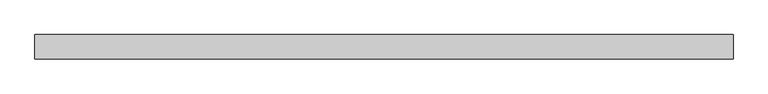
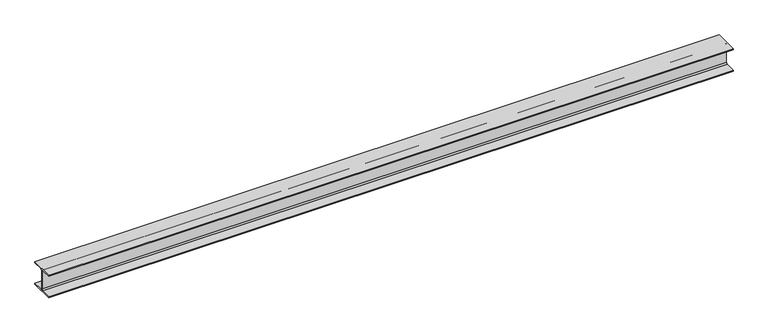
"""IFC4 building model written with IfcOpenShell, lengths in millimetres: beam geometry, 0912_Steel Framing_H-KSD3502 : H_SB_ASB_H-300x300x10x15."""

from ifc_helpers import new_model, si_unit, point, frame, frame_2d, origin, place, context, project, spatial, polyline, circle_curve, trimmed, segment, composite_curve, outline, extrude, source, transform, mapped, element, save


def beam_92893fa5(model_context):
    return source(origin(), model_context, "Body", "SweptSolid", [
        extrude(outline(composite_curve([segment(polyline([(150.0, -135.0), (150.0, -150.0), (-150.0, -150.0), (-150.0, -135.0), (-23.0, -135.0)]), True, "CONTINUOUS"), segment(trimmed(circle_curve(frame_2d((-23.0, -117.0)), 18.0), [point((-23.0, -135.0))], [point((-5.0, -117.0))], True, "CARTESIAN"), True, "CONTINUOUS"), segment(polyline([(-5.0, -117.0), (-5.0, 117.0)]), True, "CONTINUOUS"), segment(trimmed(circle_curve(frame_2d((-23.0, 117.0)), 18.0), [point((-5.0, 117.0))], [point((-23.0, 135.0))], True, "CARTESIAN"), True, "CONTINUOUS"), segment(polyline([(-23.0, 135.0), (-150.0, 135.0), (-150.0, 150.0), (150.0, 150.0), (150.0, 135.0), (23.0, 135.0)]), True, "CONTINUOUS"), segment(trimmed(circle_curve(frame_2d((23.0, 117.0)), 18.0), [point((23.0, 135.0))], [point((5.0, 117.0))], True, "CARTESIAN"), True, "CONTINUOUS"), segment(polyline([(5.0, 117.0), (5.0, -117.0)]), True, "CONTINUOUS"), segment(trimmed(circle_curve(frame_2d((23.0, -117.0)), 18.0), [point((5.0, -117.0))], [point((23.0, -135.0))], True, "CARTESIAN"), True, "CONTINUOUS"), segment(polyline([(23.0, -135.0), (150.0, -135.0)]), True, "CONTINUOUS")], self_intersect=False)), frame((-4331.4958952, 0.0, 0.0), z_axis=(1.0, 0.0, 0.0), x_axis=(0.0, 1.0, 0.0)), (0.0, 0.0, 1.0), 8594.5528849),
    ])


if __name__ == "__main__":
    model = new_model("IFC4")
    model_context = context("Model", 3, world=origin())
    ifc_project = project(units=[si_unit("LENGTHUNIT", "METRE", prefix="MILLI")], contexts=[model_context])
    site = spatial("IfcSite", under=ifc_project)
    building = spatial("IfcBuilding", under=site)
    placement = place(None, origin())
    beam_shape = beam_92893fa5(model_context)
    element("IfcBeam", 1, ObjectType="0912_Steel Framing_H-KSD3502 : H_SB_ASB_H-300x300x10x15", at=placement, inside=building, context=model_context, shape_type="MappedRepresentation", body=[
        mapped(beam_shape, transform((0.0, 0.0, 0.0), x_axis=(1.0, 0.0, 0.0), y_axis=(0.0, 1.0, 0.0), z_axis=(0.0, 0.0, 1.0))),
    ])
    save(model, "model.ifc")

# Revit data of these elements
# Type "0912_Steel Framing_H-KSD3502 : H_SB_ASB_H-300x300x10x15"
#   H_WM Code_1 = "S01AA001-00001 | Main Steel Structure Fabrication Work | Shelter/Building | Heavy Steel - Standard (Weight≥90KG/M) | Material: (   )"
#   H_WM Code_2 = "S03AA027-00001 | Main Steel Structure Erection Work | Shelter/Building | Heavy Steel (Weight≥90KG/M) | Material: (   )"
#   H_WM Code_3 = "S01AA010-00001 | Main Steel Structure Fabrication Work | Shelter/Building | Steel Painting/Coating | for Non-Fireproofed Steel Surface, Surface Preparation, Primer, Second & Final Coat | Material: (   )"
#   H_Q'ty Cal Type Tag = "SB-Q2"
#   Width = 30.0 cm
#   Web Thickness = 1.0 cm
#   Web Fillet = 1.8 cm
#   Warping Constant = 1370000.0 cm⁶
#   W = 0
#   Torsional Moment of Inertia = 77.00 cm⁴
#   Section Area = 119.8 cm²
#   Plastic Modulus weak axis = 684.0 cm³
#   Plastic Modulus strong axis = 1500.0 cm³
#   Perimeter = 1.75 m²/m
#   Nominal Weight = 94.00 kgf/m
#   Moment of Inertia weak axis = 6750.00 cm⁴
#   Moment of Inertia strong axis = 20400.00 cm⁴
#   Height = 30.0 cm
#   Flange Thickness = 1.5 cm
#   Elastic Modulus weak axis = 450.0 cm³
#   Elastic Modulus strong axis = 1360.0 cm³
#   Centroid Vertical = 15.0 cm
#   Centroid Horizontal = 15.0 cm
#   Ix = 204000000
#   Length [instance default] = 1.5240 m
#   Zx = 1500000
#   b = 0.3000 m
#   h = 0.3000 m
#   r = 0.0180 m
#   s = 0.0100 m
#   t = 0.0150 m
#   A = 0.01198 m²
#   Structural Material [instance default] = Steel, 45-345
#   Assembly Code = ""
# Element 1 (IfcBeam, "0912_Steel Framing_H-KSD3502 : H_SB_ASB_H-300x300x10x15")
#   Structural Material = none
# Materials
#   "Steel, 45-345": class "Metal", colour RGB 189 187 185, transparency 0, Description = "Steel 345 MPa", Cost = 0
